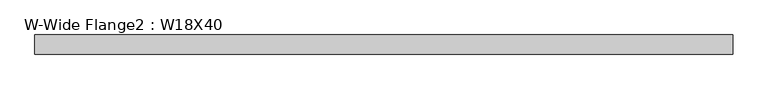
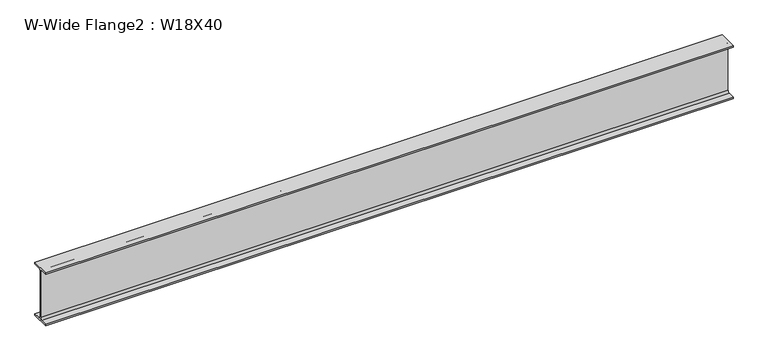
"""IFC4 building model written with IfcOpenShell, lengths in millimetres: beam geometry, W-Wide Flange2 : W18X40."""

from ifc_helpers import new_model, si_unit, point, frame, frame_2d, origin, place, context, project, spatial, polyline, circle_curve, trimmed, segment, composite_curve, outline, extrude, source, transform, mapped, element, save


def w_wide_flange2_w18x40_42c25f9a(model_context):
    return source(origin(), model_context, "Body", "SweptSolid", [
        extrude(outline(composite_curve([segment(polyline([(76.454, -213.995), (76.454, -227.33), (-76.454, -227.33), (-76.454, -213.995), (-20.828, -213.995)]), True, "CONTINUOUS"), segment(trimmed(circle_curve(frame_2d((-20.828, -197.1675)), 16.8275), [point((-20.828, -213.995))], [point((-4.0005, -197.1675))], True, "CARTESIAN"), True, "CONTINUOUS"), segment(polyline([(-4.0005, -197.1675), (-4.0005, 197.1675)]), True, "CONTINUOUS"), segment(trimmed(circle_curve(frame_2d((-20.828, 197.1675)), 16.8275), [point((-4.0005, 197.1675))], [point((-20.828, 213.995))], True, "CARTESIAN"), True, "CONTINUOUS"), segment(polyline([(-20.828, 213.995), (-76.454, 213.995), (-76.454, 227.33), (76.454, 227.33), (76.454, 213.995), (20.828, 213.995)]), True, "CONTINUOUS"), segment(trimmed(circle_curve(frame_2d((20.828, 197.1675)), 16.8275), [point((20.828, 213.995))], [point((4.0005, 197.1675))], True, "CARTESIAN"), True, "CONTINUOUS"), segment(polyline([(4.0005, 197.1675), (4.0005, -197.1675)]), True, "CONTINUOUS"), segment(trimmed(circle_curve(frame_2d((20.828, -197.1675)), 16.8275), [point((4.0005, -197.1675))], [point((20.828, -213.995))], True, "CARTESIAN"), True, "CONTINUOUS"), segment(polyline([(20.828, -213.995), (76.454, -213.995)]), True, "CONTINUOUS")], self_intersect=False)), frame((-2756.69375, 0.0, 0.0), z_axis=(1.0, 0.0, 0.0), x_axis=(0.0, 1.0, 0.0)), (0.0, 0.0, 1.0), 5570.5375),
    ])


if __name__ == "__main__":
    model = new_model("IFC4")
    model_context = context("Model", 3, world=origin())
    ifc_project = project(units=[si_unit("LENGTHUNIT", "METRE", prefix="MILLI")], contexts=[model_context])
    site = spatial("IfcSite", under=ifc_project)
    building = spatial("IfcBuilding", under=site)
    placement = place(None, origin())
    w_wide_flange2_w18x40_shape = w_wide_flange2_w18x40_42c25f9a(model_context)
    element("IfcBeam", 1, ObjectType="W-Wide Flange2 : W18X40", at=placement, inside=building, context=model_context, shape_type="MappedRepresentation", body=[
        mapped(w_wide_flange2_w18x40_shape, transform((0.0, 0.0, 0.0), x_axis=(1.0, 0.0, 0.0), y_axis=(0.0, 1.0, 0.0), z_axis=(0.0, 0.0, 1.0))),
    ])
    save(model, "model.ifc")

# Revit data of these elements
# Type "W-Wide Flange2 : W18X40"
#   Assembly Code = "B10"
#   W = 40
#   Length [instance default] = 5' - 0"
#   bf = 0' - 6.02"
#   d = 1' - 5.9"
#   k = 0' - 1 3/16"
#   k2 = 0' - 0.6625"
#   tf = 0' - 0.525"
#   tw = 0' - 0.315"
#   A = 0.0819444 SF
#   Structural Material [instance default] = Steel ASTM A992
# Element 1 (IfcBeam, "W-Wide Flange2 : W18X40")
#   Materials on its faces: "Steel ASTM A992"
# Materials
#   "Steel ASTM A992": class "Metal", colour RGB 199 199 199, transparency 0, Description = "Structural steel 50ksi", Cost = 0
